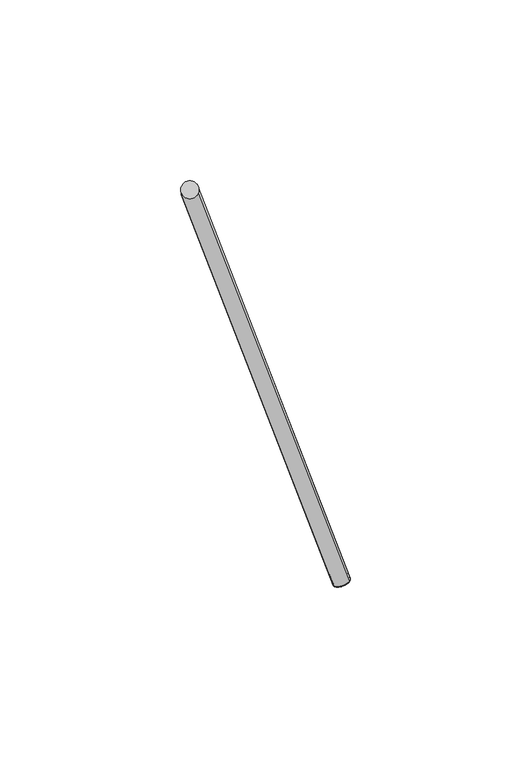
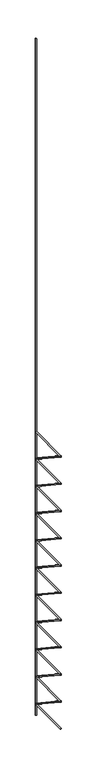
"""IFC4 building model written with IfcOpenShell, lengths in millimetres: proxy geometry, Pre-fab. (Vigota 1 - Pano 3)."""

from ifc_helpers import new_model, si_unit, point, frame, frame_2d, origin, origin_2d, place, context, project, spatial, circle_curve, trimmed, segment, composite_curve, outline, extrude, source, transform, mapped, element, save


def structural_framing_64a058b1(model_context):
    return source(origin(), model_context, "Body", "SweptSolid", [
        extrude(outline(composite_curve([segment(trimmed(circle_curve(frame_2d((-42.0, 108.0)), 2.5), [point((-39.5, 108.0))], [point((-44.5, 108.0))], False, "CARTESIAN"), True, "CONTINUOUS"), segment(trimmed(circle_curve(frame_2d((-42.0, 108.0)), 2.5), [point((-44.5, 108.0))], [point((-39.5, 108.0))], False, "CARTESIAN"), True, "CONTINUOUS")], self_intersect=False)), frame((0.0, 0.0, 39.500535), z_axis=(0.0, 0.0, 1.0), x_axis=(1.0, 0.0, 0.0)), (0.0, 0.0, 1.0), 2980.0),
        extrude(outline(composite_curve([segment(trimmed(circle_curve(origin_2d(), 2.5), [point((2.5, 0.0))], [point((-2.5, 0.0))], False, "CARTESIAN"), True, "CONTINUOUS"), segment(trimmed(circle_curve(origin_2d(), 2.5), [point((-2.5, 0.0))], [point((2.5, 0.0))], False, "CARTESIAN"), True, "CONTINUOUS")], self_intersect=False)), frame((0.0, 0.0, 29.500535), z_axis=(-0.3218603428886276, 0.8276408817707567, 0.4598004898837537), x_axis=(0.8192319205108605, -3.936835275445103e-11, 0.5734623443750141)), (0.0, 0.0, 1.0), 130.491379),
        extrude(outline(composite_curve([segment(trimmed(circle_curve(origin_2d(), 2.5), [point((2.5, 0.0))], [point((-2.5, 0.0))], False, "CARTESIAN"), True, "CONTINUOUS"), segment(trimmed(circle_curve(origin_2d(), 2.5), [point((-2.5, 0.0))], [point((2.5, 0.0))], False, "CARTESIAN"), True, "CONTINUOUS")], self_intersect=False)), frame((-42.0, 108.0, 89.500535), z_axis=(0.3218603428886276, -0.8276408817707567, 0.4598004898837537), x_axis=(0.8192319205108605, -3.936835275445103e-11, -0.5734623443750141)), (0.0, 0.0, 1.0), 130.491379),
        extrude(outline(composite_curve([segment(trimmed(circle_curve(origin_2d(), 2.5), [point((2.5, 0.0))], [point((-2.5, 0.0))], False, "CARTESIAN"), True, "CONTINUOUS"), segment(trimmed(circle_curve(origin_2d(), 2.5), [point((-2.5, 0.0))], [point((2.5, 0.0))], False, "CARTESIAN"), True, "CONTINUOUS")], self_intersect=False)), frame((0.0, 0.0, 149.500535), z_axis=(-0.3218603428886276, 0.8276408817707567, 0.4598004898837537), x_axis=(0.8192319205108605, -3.936835275445103e-11, 0.5734623443750141)), (0.0, 0.0, 1.0), 130.491379),
        extrude(outline(composite_curve([segment(trimmed(circle_curve(origin_2d(), 2.5), [point((2.5, 0.0))], [point((-2.5, 0.0))], False, "CARTESIAN"), True, "CONTINUOUS"), segment(trimmed(circle_curve(origin_2d(), 2.5), [point((-2.5, 0.0))], [point((2.5, 0.0))], False, "CARTESIAN"), True, "CONTINUOUS")], self_intersect=False)), frame((-42.0, 108.0, 209.500535), z_axis=(0.3218603428886276, -0.8276408817707567, 0.4598004898837537), x_axis=(0.8192319205108605, -3.936835275445103e-11, -0.5734623443750141)), (0.0, 0.0, 1.0), 130.491379),
        extrude(outline(composite_curve([segment(trimmed(circle_curve(origin_2d(), 2.5), [point((2.5, 0.0))], [point((-2.5, 0.0))], False, "CARTESIAN"), True, "CONTINUOUS"), segment(trimmed(circle_curve(origin_2d(), 2.5), [point((-2.5, 0.0))], [point((2.5, 0.0))], False, "CARTESIAN"), True, "CONTINUOUS")], self_intersect=False)), frame((0.0, 0.0, 269.500535), z_axis=(-0.3218603428886276, 0.8276408817707567, 0.4598004898837537), x_axis=(0.8192319205108605, -3.936835275445103e-11, 0.5734623443750141)), (0.0, 0.0, 1.0), 130.491379),
        extrude(outline(composite_curve([segment(trimmed(circle_curve(origin_2d(), 2.5), [point((2.5, 0.0))], [point((-2.5, 0.0))], False, "CARTESIAN"), True, "CONTINUOUS"), segment(trimmed(circle_curve(origin_2d(), 2.5), [point((-2.5, 0.0))], [point((2.5, 0.0))], False, "CARTESIAN"), True, "CONTINUOUS")], self_intersect=False)), frame((-42.0, 108.0, 329.500535), z_axis=(0.3218603428886276, -0.8276408817707567, 0.4598004898837537), x_axis=(0.8192319205108605, -3.936835275445103e-11, -0.5734623443750141)), (0.0, 0.0, 1.0), 130.491379),
        extrude(outline(composite_curve([segment(trimmed(circle_curve(origin_2d(), 2.5), [point((2.5, 0.0))], [point((-2.5, 0.0))], False, "CARTESIAN"), True, "CONTINUOUS"), segment(trimmed(circle_curve(origin_2d(), 2.5), [point((-2.5, 0.0))], [point((2.5, 0.0))], False, "CARTESIAN"), True, "CONTINUOUS")], self_intersect=False)), frame((0.0, 0.0, 389.500535), z_axis=(-0.3218603428886276, 0.8276408817707567, 0.4598004898837537), x_axis=(0.8192319205108605, -3.936835275445103e-11, 0.5734623443750141)), (0.0, 0.0, 1.0), 130.491379),
        extrude(outline(composite_curve([segment(trimmed(circle_curve(origin_2d(), 2.5), [point((2.5, 0.0))], [point((-2.5, 0.0))], False, "CARTESIAN"), True, "CONTINUOUS"), segment(trimmed(circle_curve(origin_2d(), 2.5), [point((-2.5, 0.0))], [point((2.5, 0.0))], False, "CARTESIAN"), True, "CONTINUOUS")], self_intersect=False)), frame((-42.0, 108.0, 449.500535), z_axis=(0.3218603428886276, -0.8276408817707567, 0.4598004898837537), x_axis=(0.8192319205108605, -3.936835275445103e-11, -0.5734623443750141)), (0.0, 0.0, 1.0), 130.491379),
        extrude(outline(composite_curve([segment(trimmed(circle_curve(origin_2d(), 2.5), [point((2.5, 0.0))], [point((-2.5, 0.0))], False, "CARTESIAN"), True, "CONTINUOUS"), segment(trimmed(circle_curve(origin_2d(), 2.5), [point((-2.5, 0.0))], [point((2.5, 0.0))], False, "CARTESIAN"), True, "CONTINUOUS")], self_intersect=False)), frame((0.0, 0.0, 509.500535), z_axis=(-0.3218603428886276, 0.8276408817707567, 0.4598004898837537), x_axis=(0.8192319205108605, -3.936835275445103e-11, 0.5734623443750141)), (0.0, 0.0, 1.0), 130.491379),
        extrude(outline(composite_curve([segment(trimmed(circle_curve(origin_2d(), 2.5), [point((2.5, 0.0))], [point((-2.5, 0.0))], False, "CARTESIAN"), True, "CONTINUOUS"), segment(trimmed(circle_curve(origin_2d(), 2.5), [point((-2.5, 0.0))], [point((2.5, 0.0))], False, "CARTESIAN"), True, "CONTINUOUS")], self_intersect=False)), frame((-42.0, 108.0, 569.500535), z_axis=(0.3218603428886276, -0.8276408817707567, 0.4598004898837537), x_axis=(0.8192319205108605, -3.936835275445103e-11, -0.5734623443750141)), (0.0, 0.0, 1.0), 130.491379),
        extrude(outline(composite_curve([segment(trimmed(circle_curve(origin_2d(), 2.5), [point((2.5, 0.0))], [point((-2.5, 0.0))], False, "CARTESIAN"), True, "CONTINUOUS"), segment(trimmed(circle_curve(origin_2d(), 2.5), [point((-2.5, 0.0))], [point((2.5, 0.0))], False, "CARTESIAN"), True, "CONTINUOUS")], self_intersect=False)), frame((0.0, 0.0, 629.500535), z_axis=(-0.3218603428886276, 0.8276408817707567, 0.4598004898837537), x_axis=(0.8192319205108605, -3.936835275445103e-11, 0.5734623443750141)), (0.0, 0.0, 1.0), 130.491379),
        extrude(outline(composite_curve([segment(trimmed(circle_curve(origin_2d(), 2.5), [point((2.5, 0.0))], [point((-2.5, 0.0))], False, "CARTESIAN"), True, "CONTINUOUS"), segment(trimmed(circle_curve(origin_2d(), 2.5), [point((-2.5, 0.0))], [point((2.5, 0.0))], False, "CARTESIAN"), True, "CONTINUOUS")], self_intersect=False)), frame((-42.0, 108.0, 689.500535), z_axis=(0.3218603428886276, -0.8276408817707567, 0.4598004898837537), x_axis=(0.8192319205108605, -3.936835275445103e-11, -0.5734623443750141)), (0.0, 0.0, 1.0), 130.491379),
        extrude(outline(composite_curve([segment(trimmed(circle_curve(origin_2d(), 2.5), [point((2.5, 0.0))], [point((-2.5, 0.0))], False, "CARTESIAN"), True, "CONTINUOUS"), segment(trimmed(circle_curve(origin_2d(), 2.5), [point((-2.5, 0.0))], [point((2.5, 0.0))], False, "CARTESIAN"), True, "CONTINUOUS")], self_intersect=False)), frame((0.0, 0.0, 749.500535), z_axis=(-0.3218603428886276, 0.8276408817707567, 0.4598004898837537), x_axis=(0.8192319205108605, -3.936835275445103e-11, 0.5734623443750141)), (0.0, 0.0, 1.0), 130.491379),
        extrude(outline(composite_curve([segment(trimmed(circle_curve(origin_2d(), 2.5), [point((2.5, 0.0))], [point((-2.5, 0.0))], False, "CARTESIAN"), True, "CONTINUOUS"), segment(trimmed(circle_curve(origin_2d(), 2.5), [point((-2.5, 0.0))], [point((2.5, 0.0))], False, "CARTESIAN"), True, "CONTINUOUS")], self_intersect=False)), frame((-42.0, 108.0, 809.500535), z_axis=(0.3218603428886276, -0.8276408817707567, 0.4598004898837537), x_axis=(0.8192319205108605, -3.936835275445103e-11, -0.5734623443750141)), (0.0, 0.0, 1.0), 130.491379),
        extrude(outline(composite_curve([segment(trimmed(circle_curve(origin_2d(), 2.5), [point((2.5, 0.0))], [point((-2.5, 0.0))], False, "CARTESIAN"), True, "CONTINUOUS"), segment(trimmed(circle_curve(origin_2d(), 2.5), [point((-2.5, 0.0))], [point((2.5, 0.0))], False, "CARTESIAN"), True, "CONTINUOUS")], self_intersect=False)), frame((0.0, 0.0, 869.500535), z_axis=(-0.3218603428886276, 0.8276408817707567, 0.4598004898837537), x_axis=(0.8192319205108605, -3.936835275445103e-11, 0.5734623443750141)), (0.0, 0.0, 1.0), 130.491379),
        extrude(outline(composite_curve([segment(trimmed(circle_curve(origin_2d(), 2.5), [point((2.5, 0.0))], [point((-2.5, 0.0))], False, "CARTESIAN"), True, "CONTINUOUS"), segment(trimmed(circle_curve(origin_2d(), 2.5), [point((-2.5, 0.0))], [point((2.5, 0.0))], False, "CARTESIAN"), True, "CONTINUOUS")], self_intersect=False)), frame((-42.0, 108.0, 929.500535), z_axis=(0.3218603428886276, -0.8276408817707567, 0.4598004898837537), x_axis=(0.8192319205108605, -3.936835275445103e-11, -0.5734623443750141)), (0.0, 0.0, 1.0), 130.491379),
        extrude(outline(composite_curve([segment(trimmed(circle_curve(origin_2d(), 2.5), [point((2.5, 0.0))], [point((-2.5, 0.0))], False, "CARTESIAN"), True, "CONTINUOUS"), segment(trimmed(circle_curve(origin_2d(), 2.5), [point((-2.5, 0.0))], [point((2.5, 0.0))], False, "CARTESIAN"), True, "CONTINUOUS")], self_intersect=False)), frame((0.0, 0.0, 989.500535), z_axis=(-0.3218603428886276, 0.8276408817707567, 0.4598004898837537), x_axis=(0.8192319205108605, -3.936835275445103e-11, 0.5734623443750141)), (0.0, 0.0, 1.0), 130.491379),
        extrude(outline(composite_curve([segment(trimmed(circle_curve(origin_2d(), 2.5), [point((2.5, 0.0))], [point((-2.5, 0.0))], False, "CARTESIAN"), True, "CONTINUOUS"), segment(trimmed(circle_curve(origin_2d(), 2.5), [point((-2.5, 0.0))], [point((2.5, 0.0))], False, "CARTESIAN"), True, "CONTINUOUS")], self_intersect=False)), frame((-42.0, 108.0, 1049.500535), z_axis=(0.3218603428886276, -0.8276408817707567, 0.4598004898837537), x_axis=(0.8192319205108605, -3.936835275445103e-11, -0.5734623443750141)), (0.0, 0.0, 1.0), 130.491379),
        extrude(outline(composite_curve([segment(trimmed(circle_curve(origin_2d(), 2.5), [point((2.5, 0.0))], [point((-2.5, 0.0))], False, "CARTESIAN"), True, "CONTINUOUS"), segment(trimmed(circle_curve(origin_2d(), 2.5), [point((-2.5, 0.0))], [point((2.5, 0.0))], False, "CARTESIAN"), True, "CONTINUOUS")], self_intersect=False)), frame((0.0, 0.0, 1109.500535), z_axis=(-0.3218603428886276, 0.8276408817707567, 0.4598004898837537), x_axis=(0.8192319205108605, -3.936835275445103e-11, 0.5734623443750141)), (0.0, 0.0, 1.0), 130.491379),
        extrude(outline(composite_curve([segment(trimmed(circle_curve(origin_2d(), 2.5), [point((2.5, 0.0))], [point((-2.5, 0.0))], False, "CARTESIAN"), True, "CONTINUOUS"), segment(trimmed(circle_curve(origin_2d(), 2.5), [point((-2.5, 0.0))], [point((2.5, 0.0))], False, "CARTESIAN"), True, "CONTINUOUS")], self_intersect=False)), frame((-42.0, 108.0, 1169.500535), z_axis=(0.3218603428886276, -0.8276408817707567, 0.4598004898837537), x_axis=(0.8192319205108605, -3.936835275445103e-11, -0.5734623443750141)), (0.0, 0.0, 1.0), 130.491379),
        extrude(outline(composite_curve([segment(trimmed(circle_curve(origin_2d(), 2.5), [point((2.5, 0.0))], [point((-2.5, 0.0))], False, "CARTESIAN"), True, "CONTINUOUS"), segment(trimmed(circle_curve(origin_2d(), 2.5), [point((-2.5, 0.0))], [point((2.5, 0.0))], False, "CARTESIAN"), True, "CONTINUOUS")], self_intersect=False)), frame((0.0, 0.0, 1229.500535), z_axis=(-0.3218603428886276, 0.8276408817707567, 0.4598004898837537), x_axis=(0.8192319205108605, -3.936835275445103e-11, 0.5734623443750141)), (0.0, 0.0, 1.0), 130.491379),
    ])


if __name__ == "__main__":
    model = new_model("IFC4")
    model_context = context("Model", 3, world=origin())
    ifc_project = project(units=[si_unit("LENGTHUNIT", "METRE", prefix="MILLI")], contexts=[model_context])
    site = spatial("IfcSite", under=ifc_project)
    building = spatial("IfcBuilding", under=site)
    placement = place(None, origin())
    structural_framing_shape = structural_framing_64a058b1(model_context)
    element("IfcBuildingElementProxy", 1, Name="Pre-fab. (Vigota 1 - Pano 3)", ObjectType="Pre-fab. (Vigota 1 - Pano 3)", at=placement, inside=building, context=model_context, shape_type="MappedRepresentation", body=[
        mapped(structural_framing_shape, transform((0.0, 0.0, 0.0), x_axis=(1.0, 0.0, 0.0), y_axis=(0.0, 1.0, 0.0), z_axis=(0.0, 0.0, 1.0))),
    ])
    save(model, "model.ifc")

# Revit data of these elements
# Element 1 (IfcBuildingElementProxy, "Pre-fab. (Vigota 1 - Pano 3)")
#   Materials on its faces: "Aço"
# Materials
#   "Aço": class "Metal", colour RGB 120 120 120, transparency 0, Description = "Aço estrutural A36 grau, ASTM B, acabamento laminado", Cost = 0
